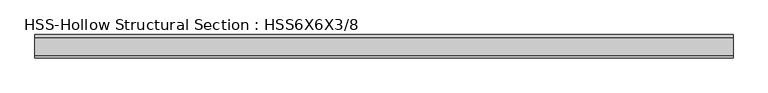
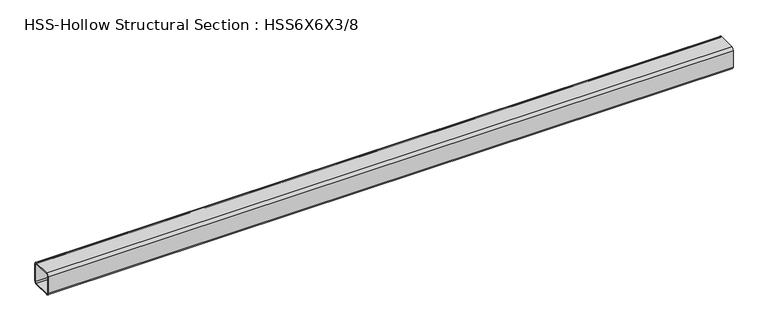
"""IFC4 building model written with IfcOpenShell, lengths in millimetres: member geometry, HSS-Hollow Structural Section : HSS6X6X3/8."""

from ifc_helpers import new_model, si_unit, point, frame, frame_2d, origin, place, context, project, spatial, polyline, circle_curve, trimmed, segment, composite_curve, outline, extrude, source, transform, mapped, element, save


def hss_hollow_structural_section_hss6x6x3_8_529a6282(model_context):
    return source(origin(), model_context, "Body", "SweptSolid", [
        extrude(outline(composite_curve([segment(polyline([(76.2, 58.4708), (76.2, -58.4708)]), True, "CONTINUOUS"), segment(trimmed(circle_curve(frame_2d((58.4708, -58.4708)), 17.7292), [point((76.2, -58.4708))], [point((58.4708, -76.2))], False, "CARTESIAN"), True, "CONTINUOUS"), segment(polyline([(58.4708, -76.2), (-58.4708, -76.2)]), True, "CONTINUOUS"), segment(trimmed(circle_curve(frame_2d((-58.4708, -58.4708)), 17.7292), [point((-58.4708, -76.2))], [point((-76.2, -58.4708))], False, "CARTESIAN"), True, "CONTINUOUS"), segment(polyline([(-76.2, -58.4708), (-76.2, 58.4708)]), True, "CONTINUOUS"), segment(trimmed(circle_curve(frame_2d((-58.4708, 58.4708)), 17.7292), [point((-76.2, 58.4708))], [point((-58.4708, 76.2))], False, "CARTESIAN"), True, "CONTINUOUS"), segment(polyline([(-58.4708, 76.2), (58.4708, 76.2)]), True, "CONTINUOUS"), segment(trimmed(circle_curve(frame_2d((58.4708, 58.4708)), 17.7292), [point((58.4708, 76.2))], [point((76.2, 58.4708))], False, "CARTESIAN"), True, "CONTINUOUS")], self_intersect=False), holes=[composite_curve([segment(trimmed(circle_curve(frame_2d((-58.4708, 58.4708)), 8.8646), [point((-58.4708, 67.3354))], [point((-67.3354, 58.4708))], True, "CARTESIAN"), True, "CONTINUOUS"), segment(polyline([(-67.3354, 58.4708), (-67.3354, -58.4708)]), True, "CONTINUOUS"), segment(trimmed(circle_curve(frame_2d((-58.4708, -58.4708)), 8.8646), [point((-67.3354, -58.4708))], [point((-58.4708, -67.3354))], True, "CARTESIAN"), True, "CONTINUOUS"), segment(polyline([(-58.4708, -67.3354), (58.4708, -67.3354)]), True, "CONTINUOUS"), segment(trimmed(circle_curve(frame_2d((58.4708, -58.4708)), 8.8646), [point((58.4708, -67.3354))], [point((67.3354, -58.4708))], True, "CARTESIAN"), True, "CONTINUOUS"), segment(polyline([(67.3354, -58.4708), (67.3354, 58.4708)]), True, "CONTINUOUS"), segment(trimmed(circle_curve(frame_2d((58.4708, 58.4708)), 8.8646), [point((67.3354, 58.4708))], [point((58.4708, 67.3354))], True, "CARTESIAN"), True, "CONTINUOUS"), segment(polyline([(58.4708, 67.3354), (-58.4708, 67.3354)]), True, "CONTINUOUS")], self_intersect=False)]), frame((-2343.8359473, 0.0, 0.0), z_axis=(1.0, 0.0, 0.0), x_axis=(0.0, 1.0, 0.0)), (0.0, 0.0, 1.0), 4563.6191827),
    ])


if __name__ == "__main__":
    model = new_model("IFC4")
    model_context = context("Model", 3, world=origin())
    ifc_project = project(units=[si_unit("LENGTHUNIT", "METRE", prefix="MILLI")], contexts=[model_context])
    site = spatial("IfcSite", under=ifc_project)
    building = spatial("IfcBuilding", under=site)
    placement = place(None, origin())
    hss_hollow_structural_section_hss6x6x3_8_shape = hss_hollow_structural_section_hss6x6x3_8_529a6282(model_context)
    element("IfcMember", 1, ObjectType="HSS-Hollow Structural Section : HSS6X6X3/8", at=placement, inside=building, context=model_context, shape_type="MappedRepresentation", body=[
        mapped(hss_hollow_structural_section_hss6x6x3_8_shape, transform((0.0, 0.0, 0.0), x_axis=(1.0, 0.0, 0.0), y_axis=(0.0, 1.0, 0.0), z_axis=(0.0, 0.0, 1.0))),
    ])
    save(model, "model.ifc")

# Revit data of these elements
# Type "HSS-Hollow Structural Section : HSS6X6X3/8"
#   Assembly Code = "B10"
#   Shape = "Square"
#   W = 27.4
#   Ht = 0' - 6"
#   Length [instance default] = 5' - 0"
#   b = 0' - 6"
#   kr = 0' - 0.698"
#   t = 0' - 0.349"
#   A = 0.0526389 SF
#   Structural Material [instance default] = Steel ASTM A500, Grade B, Rectangular and Square
# Element 1 (IfcMember, "HSS-Hollow Structural Section : HSS6X6X3/8")
#   Materials on its faces: "Steel ASTM A500, Grade B, Rectangular and Square"
# Materials
#   "Steel ASTM A500, Grade B, Rectangular and Square": class "Metal", colour RGB 199 199 199, transparency 0, Description = "Carbon steel", Cost = 0
